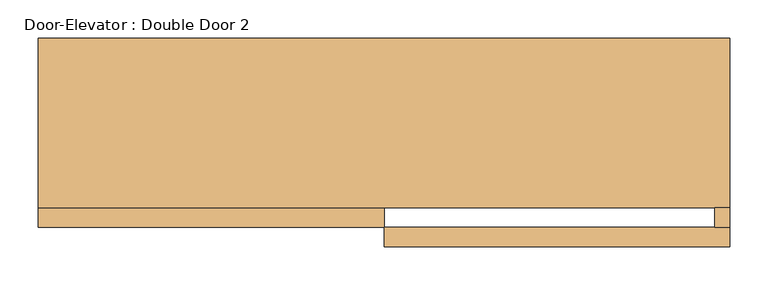
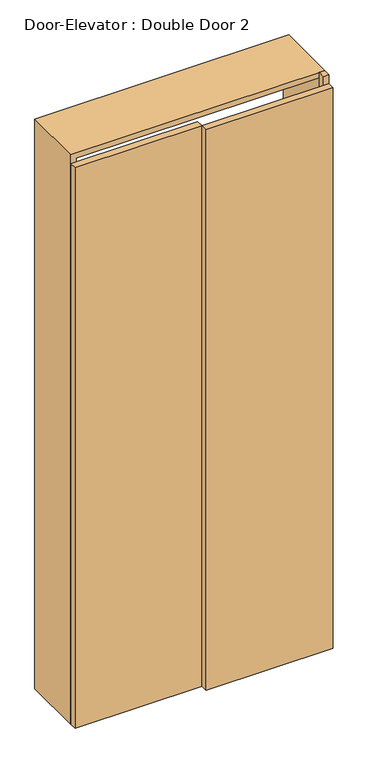
"""IFC4 building model written with IfcOpenShell, lengths in millimetres: door geometry, Door-Elevator : Double Door 2."""

from ifc_helpers import new_model, si_unit, frame, origin, origin_with_axes, place, context, project, spatial, polyline, outline, extrude, source, transform, mapped, element, save


def door_elevator_double_door_2_208132c5(model_context):
    return source(origin(), model_context, "Body", "SweptSolid", [
        extrude(outline(polyline([(450.0, -157.15), (450.0, -182.55), (0.0, -182.55), (0.0, -157.15), (450.0, -157.15)])), origin_with_axes(), (0.0, 0.0, 1.0), 2100.0),
        extrude(outline(polyline([(0.0, -131.75), (0.0, -157.15), (-450.0, -157.15), (-450.0, -131.75), (0.0, -131.75)])), origin_with_axes(), (0.0, 0.0, 1.0), 2100.0),
        extrude(outline(polyline([(450.0, -131.75), (450.0, -157.15), (430.95, -157.15), (430.95, -131.75), (450.0, -131.75)])), origin_with_axes(), (0.0, 0.0, 1.0), 2133.6),
        extrude(outline(polyline([(0.0, -430.95), (2114.55, -430.95), (2114.55, 430.95), (0.0, 430.95), (0.0, 450.0), (2133.6, 450.0), (2133.6, -450.0), (0.0, -450.0), (0.0, -430.95)])), frame((0.0, -131.75, 0.0), z_axis=(0.0, 1.0, 0.0), x_axis=(0.0, 0.0, 1.0)), (0.0, 0.0, 1.0), 220.65),
    ])


if __name__ == "__main__":
    model = new_model("IFC4")
    model_context = context("Model", 3, world=origin())
    ifc_project = project(units=[si_unit("LENGTHUNIT", "METRE", prefix="MILLI")], contexts=[model_context])
    site = spatial("IfcSite", under=ifc_project)
    building = spatial("IfcBuilding", under=site)
    placement = place(None, origin())
    door_elevator_double_door_2_shape = door_elevator_double_door_2_208132c5(model_context)
    element("IfcDoor", 1, ObjectType="Door-Elevator : Double Door 2", at=placement, inside=building, context=model_context, shape_type="MappedRepresentation", body=[
        mapped(door_elevator_double_door_2_shape, transform((0.0, 0.0, 0.0), x_axis=(1.0, 0.0, 0.0), y_axis=(0.0, 1.0, 0.0), z_axis=(0.0, 0.0, 1.0))),
    ])
    save(model, "model.ifc")

# Revit data of these elements
# Type "Door-Elevator : Double Door 2"
#   Type Mark = "EX1-59"
#   P_WWSKU = ""
#   Filter Visibiilty = "Existing Elevator"
#   Analytic Construction = "<None>"
#   Trim Projection = 12.7 mm
#   Thickness = 25.4 mm
#   Height = 2100 mm
#   Trim Width = 19.05 mm
#   Width = 900 mm
#   Door_Quad = 225 mm
#   Door_Double = 450 mm
#   Cab Width = 1828.8 mm
#   Cab Offset [instance default] = 0 mm
#   Cab Depth = 1828.8 mm
#   _factor4 = 4
#   _factor2 = 2
#   WW-HardwareSet [instance default] = 0
#   Simple Plan = yes
#   Quad = no
#   Plan Lines [instance default] = yes
#   Double = yes
#   Panel Type = element 9002524
#   Type Comments = ""
#   Keynote = ""
#   Function = (empty or 0)
#   Wall Closure = (empty or 0)
#   Assembly Code = ""
# Element 1 (IfcDoor, "Door-Elevator : Double Door 2")
#   Materials on its faces: "WW-EC-RGB-White"
# Materials
#   "WW-EC-RGB-White": class "Generic", colour RGB 255 255 255, transparency 0, Comments = "If region requests off-white, swith asset color to RGB 231-228-220", Description = "Generic Color", Cost = 0
